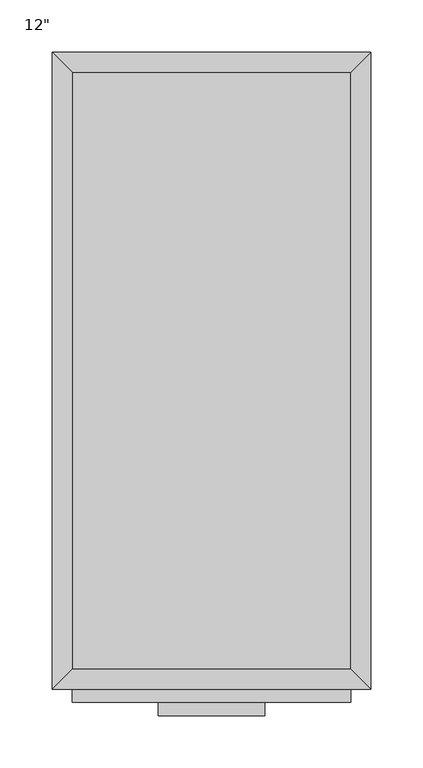
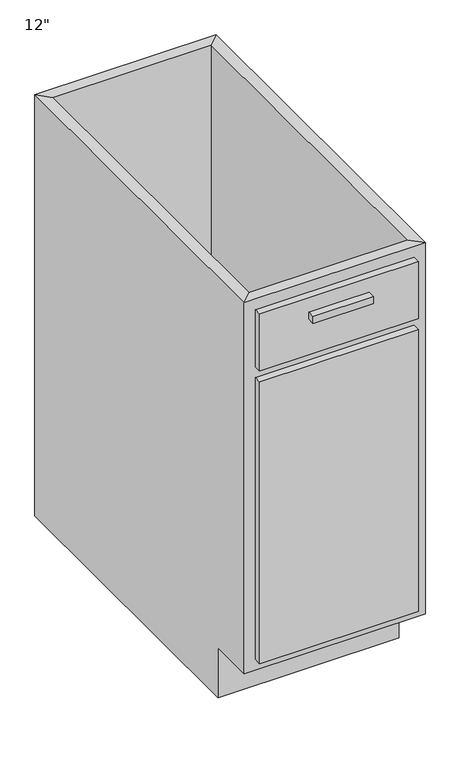
"""IFC4 building model written with IfcOpenShell, lengths in millimetres: furniture geometry."""

import ifcopenshell
import ifcopenshell.guid

model = None  # the IFC model being written
_history = None  # IfcOwnerHistory: only IFC2X3 demands one
_inside = {}  # id of a spatial element -> (the spatial element, [elements in it])
_under = {}  # id of a project, library or spatial element -> (it, [spatial elements below it])
_declared = {}  # id of a project -> (the project, [libraries it declares])
_typed = {}  # id of a type object -> (the type object, [elements of that type])
_made_of = {}  # id of a material, layer set ... -> (it, [elements and type objects made of it])


def new_model(schema):
    """Start an empty IFC model of exactly this schema.

    Asked for "IFC4X3", IfcOpenShell would pick the latest addendum, in which some entities
    have other attributes; the version numbers below select the first issue.
    IFC2X3 requires an IfcOwnerHistory on every rooted entity: one is made here for all.
    """
    global model, _history
    if schema == "IFC4X3":
        model = ifcopenshell.file(schema_version=(4, 3, 0, 0))
    else:
        model = ifcopenshell.file(schema=schema)
    _inside.clear()
    _under.clear()
    _declared.clear()
    _typed.clear()
    _made_of.clear()
    _history = None
    if model.schema == "IFC2X3":
        org = make("IfcOrganization", Name="unknown")
        user = make(
            "IfcPersonAndOrganization",
            ThePerson=make("IfcPerson", FamilyName="unknown"),
            TheOrganization=org,
        )
        app = make(
            "IfcApplication",
            ApplicationDeveloper=org,
            Version="unknown",
            ApplicationFullName="unknown",
            ApplicationIdentifier="unknown",
        )
        _history = make(
            "IfcOwnerHistory",
            OwningUser=user,
            OwningApplication=app,
            ChangeAction="ADDED",
            CreationDate=0,
        )
    return model


def make(cls, **values):
    """One entity of the class cls with the attributes given. An attribute that is None is left unset."""
    return model.create_entity(
        cls, **{name: value for name, value in values.items() if value is not None}
    )


def rooted(cls, **values):
    """An entity with a GlobalId (a new one), such as an element, a storey or a relation."""
    return make(cls, GlobalId=ifcopenshell.guid.new(), OwnerHistory=_history, **values)


def si_unit(unit_type, name, prefix=None):
    """IfcSIUnit, for example si_unit("LENGTHUNIT", "METRE", prefix="MILLI")."""
    return make("IfcSIUnit", UnitType=unit_type, Prefix=prefix, Name=name)


def assignment(units):
    """IfcUnitAssignment: the units of a project."""
    return None if units is None else make("IfcUnitAssignment", Units=units)


def point(xyz):
    """IfcCartesianPoint."""
    return None if xyz is None else make("IfcCartesianPoint", Coordinates=xyz)


def direction(xyz):
    """IfcDirection."""
    return None if xyz is None else make("IfcDirection", DirectionRatios=xyz)


def frame(location, z_axis=None, x_axis=None):
    """IfcAxis2Placement3D, a coordinate frame: its origin and axes. An axis left out is left unset."""
    return make(
        "IfcAxis2Placement3D",
        Location=point(location),
        Axis=direction(z_axis),
        RefDirection=direction(x_axis),
    )


def origin():
    """The frame at (0, 0, 0) with its axes left unset."""
    return frame((0.0, 0.0, 0.0))


def place(relative_to, where):
    """IfcLocalPlacement: puts the frame where relative to a parent placement (None: the world)."""
    return make(
        "IfcLocalPlacement", PlacementRelTo=relative_to, RelativePlacement=where
    )


def context(
    kind, dimensions, precision=None, world=None, true_north=None, identifier=None
):
    """IfcGeometricRepresentationContext, for example the 3D "Model" context."""
    return make(
        "IfcGeometricRepresentationContext",
        ContextIdentifier=identifier,
        ContextType=kind,
        CoordinateSpaceDimension=dimensions,
        Precision=precision,
        WorldCoordinateSystem=world,
        TrueNorth=true_north,
    )


def project(units=None, contexts=None):
    """IfcProject with its units and contexts."""
    return rooted(
        "IfcProject",
        Name="project",
        RepresentationContexts=contexts,
        UnitsInContext=assignment(units),
    )


def spatial(cls, under=None, at=None, **own):
    """A site, building, storey or space (cls), placed at a placement, below another one or the project."""
    s = rooted(cls, ObjectPlacement=at, **own)
    if under is not None:
        _under.setdefault(under.id(), (under, []))[1].append(s)
    return s


def polyline(points):
    """IfcPolyline through the points."""
    return make("IfcPolyline", Points=[point(p) for p in points])


def outline(outer, holes=None, kind="AREA"):
    """IfcArbitraryClosedProfileDef: a profile drawn as a closed curve; with holes, ...WithVoids."""
    if holes is None:
        return make("IfcArbitraryClosedProfileDef", ProfileType=kind, OuterCurve=outer)
    return make(
        "IfcArbitraryProfileDefWithVoids",
        ProfileType=kind,
        OuterCurve=outer,
        InnerCurves=holes,
    )


def extrude(swept, where, along, depth):
    """IfcExtrudedAreaSolid: the profile swept, set in the frame where, extruded along a direction by depth."""
    return make(
        "IfcExtrudedAreaSolid",
        SweptArea=swept,
        Position=where,
        ExtrudedDirection=direction(along),
        Depth=depth,
    )


def faces_of(points, faces, orient=None, outer=None):
    """IfcFace entities. A face is a list of loops; a loop is a list of indices into points, from 0.

    orient and outer hold one flag for each loop. By default every Orientation is true, the
    first loop of a face is its IfcFaceOuterBound and the others are IfcFaceBound.
    """
    made = []
    for i, loops in enumerate(faces):
        bounds = []
        for j, loop in enumerate(loops):
            is_outer = j == 0 if outer is None else outer[i][j]
            bounds.append(
                make(
                    "IfcFaceOuterBound" if is_outer else "IfcFaceBound",
                    Bound=make("IfcPolyLoop", Polygon=[points[k] for k in loop]),
                    Orientation=True if orient is None else orient[i][j],
                )
            )
        made.append(make("IfcFace", Bounds=bounds))
    return made


def faceted_brep(points, faces, orient=None, outer=None, voids=None):
    """IfcFacetedBrep: a solid bounded by flat faces; with voids (closed shells), ...WithVoids."""
    shared = [point(p) for p in points]
    hull = make("IfcClosedShell", CfsFaces=faces_of(shared, faces, orient, outer))
    if voids is None:
        return make("IfcFacetedBrep", Outer=hull)
    return make(
        "IfcFacetedBrepWithVoids",
        Outer=hull,
        Voids=[
            make(cls, CfsFaces=faces_of(shared, fs, o, b)) for cls, fs, o, b in voids
        ],
    )


def shape(context_of_items, identifier, shape_type, items):
    """IfcShapeRepresentation: the items that make up one representation, for example the "Body"."""
    return make(
        "IfcShapeRepresentation",
        ContextOfItems=context_of_items,
        RepresentationIdentifier=identifier,
        RepresentationType=shape_type,
        Items=items,
    )


def source(mapping_origin, context_of_items, identifier, shape_type, items):
    """IfcRepresentationMap: a shape defined once, which mapped items show again and again."""
    return make(
        "IfcRepresentationMap",
        MappingOrigin=mapping_origin,
        MappedRepresentation=shape(context_of_items, identifier, shape_type, items),
    )


def transform(
    local_origin,
    x_axis=None,
    y_axis=None,
    z_axis=None,
    scale=None,
    scale2=None,
    scale3=None,
    uniform=True,
):
    """IfcCartesianTransformationOperator3D, or its non-uniform kind. x_axis, y_axis, z_axis: its Axis1, 2, 3."""
    if uniform:
        return make(
            "IfcCartesianTransformationOperator3D",
            Axis1=direction(x_axis),
            Axis2=direction(y_axis),
            LocalOrigin=point(local_origin),
            Scale=scale,
            Axis3=direction(z_axis),
        )
    return make(
        "IfcCartesianTransformationOperator3DnonUniform",
        Axis1=direction(x_axis),
        Axis2=direction(y_axis),
        LocalOrigin=point(local_origin),
        Scale=scale,
        Axis3=direction(z_axis),
        Scale2=scale2,
        Scale3=scale3,
    )


def mapped(mapping_source, mapping_target):
    """IfcMappedItem: shows the shape of a source again, moved by a transform."""
    return make(
        "IfcMappedItem", MappingSource=mapping_source, MappingTarget=mapping_target
    )


def made_of(thing, what):
    """Note that an element or type object is made of a material, layer set ...; save() writes the relation."""
    if what is not None:
        _made_of.setdefault(what.id(), (what, []))[1].append(thing)
    return thing


def element(
    cls,
    number,
    at=None,
    inside=None,
    cuts=None,
    type_object=None,
    material=None,
    context=None,
    identifier="Body",
    shape_type=None,
    held_by="IfcProductDefinitionShape",
    body=None,
    shapes=None,
    **own,
):
    """One element of the class cls, such as IfcWall. Its Tag is "e" and its number.

    at: its placement. inside: the storey or other place that contains it. cuts: it is an
    opening in that element (IfcRelVoidsElement). A single representation is given by context,
    identifier, shape_type and body (its items); several are given by shapes. held_by: the class
    of the entity that holds the representations. save() writes the other relations.
    """
    e = rooted(cls, Tag="e%d" % number, ObjectPlacement=at, **own)
    if body is not None:
        shapes = [shape(context, identifier, shape_type, body)]
    if shapes is not None:
        e.Representation = make(held_by, Representations=shapes)
    if inside is not None:
        _inside.setdefault(inside.id(), (inside, []))[1].append(e)
    if cuts is not None:
        rooted(
            "IfcRelVoidsElement", RelatingBuildingElement=cuts, RelatedOpeningElement=e
        )
    if type_object is not None:
        _typed.setdefault(type_object.id(), (type_object, []))[1].append(e)
    return made_of(e, material)


def aggregate(whole, parts):
    """IfcRelAggregates: a whole, such as a stair, and the parts it consists of."""
    return rooted("IfcRelAggregates", RelatingObject=whole, RelatedObjects=parts)


def save(model, path):
    """Write the relations noted so far, then the file.

    IfcRelAggregates (storeys below a building ...), IfcRelContainedInSpatialStructure (elements
    in a storey), IfcRelDefinesByType, IfcRelAssociatesMaterial and IfcRelDeclares: one each for
    every whole, place, type object, material and project.
    """
    for whole, parts in _under.values():
        aggregate(whole, parts)
    for where, things in _inside.values():
        rooted(
            "IfcRelContainedInSpatialStructure",
            RelatedElements=things,
            RelatingStructure=where,
        )
    for kind, things in _typed.values():
        rooted("IfcRelDefinesByType", RelatedObjects=things, RelatingType=kind)
    for what, things in _made_of.values():
        rooted("IfcRelAssociatesMaterial", RelatedObjects=things, RelatingMaterial=what)
    for by, libraries in _declared.values():
        rooted("IfcRelDeclares", RelatingContext=by, RelatedDefinitions=libraries)
    model.write(path)


def furniture_d3494f9b(model_context):
    return source(origin(), model_context, "Body", "SolidModel", [
        faceted_brep([(152.0877049, -590.55, 749.3), (152.0877049, -590.55, 88.9), (-114.6122951, -590.55, 88.9), (-114.6122951, -590.55, 749.3), (-133.6622951, -609.6, 749.3), (171.1377049, -609.6, 749.3), (-133.6622951, -609.6, 88.9), (171.1377049, -609.6, 88.9), (-114.6122951, -533.4, 88.9), (-114.6122951, -19.05, 88.9), (-114.6122951, -19.05, 749.3), (-133.6622951, 0.0, 749.3), (-133.6622951, 0.0, 0.0), (-133.6622951, -533.4, 0.0), (-133.6622951, -533.4, 88.9), (152.0877049, -19.05, 88.9), (152.0877049, -19.05, 749.3), (171.1377049, 0.0, 749.3), (171.1377049, 0.0, 0.0), (152.0877049, -533.4, 88.9), (171.1377049, -533.4, 88.9), (171.1377049, -533.4, 0.0)], [[[0, 1, 2, 3]], [[0, 3, 4, 5]], [[5, 4, 6, 7]], [[2, 1, 7, 6]], [[3, 2, 8, 9, 10]], [[4, 3, 10, 11]], [[6, 4, 11, 12, 13, 14]], [[2, 6, 14, 8]], [[10, 9, 15, 16]], [[11, 10, 16, 17]], [[12, 11, 17, 18]], [[1, 0, 16, 15, 19]], [[0, 5, 17, 16]], [[5, 7, 20, 21, 18, 17]], [[7, 1, 19, 20]], [[8, 19, 15, 9]], [[18, 21, 13, 12]], [[13, 21, 20, 19, 8, 14]]]),
        extrude(outline(polyline([(152.0877049, -19.05), (152.0877049, -590.55), (-114.6122951, -590.55), (-114.6122951, -19.05), (152.0877049, -19.05)])), frame((0.0, 0.0, 88.9), z_axis=(0.0, 0.0, 1.0), x_axis=(1.0, 0.0, 0.0)), (0.0, 0.0, 1.0), 19.05),
        extrude(outline(polyline([(152.0877049, -622.3), (-114.6122951, -622.3), (-114.6122951, -609.6), (152.0877049, -609.6), (152.0877049, -622.3)])), frame((0.0, 0.0, 628.65), z_axis=(0.0, 0.0, 1.0), x_axis=(1.0, 0.0, 0.0)), (0.0, 0.0, 1.0), 101.6),
        extrude(outline(polyline([(152.0877049, -622.3), (-114.6122951, -622.3), (-114.6122951, -609.6), (152.0877049, -609.6), (152.0877049, -622.3)])), frame((0.0, 0.0, 107.95), z_axis=(0.0, 0.0, 1.0), x_axis=(1.0, 0.0, 0.0)), (0.0, 0.0, 1.0), 501.65),
        extrude(outline(polyline([(69.5377049, -635.0), (-32.0622951, -635.0), (-32.0622951, -622.3), (69.5377049, -622.3), (69.5377049, -635.0)])), frame((0.0, 0.0, 692.15), z_axis=(0.0, 0.0, 1.0), x_axis=(1.0, 0.0, 0.0)), (0.0, 0.0, 1.0), 12.7),
    ])


if __name__ == "__main__":
    model = new_model("IFC4")
    model_context = context("Model", 3, world=origin())
    ifc_project = project(units=[si_unit("LENGTHUNIT", "METRE", prefix="MILLI")], contexts=[model_context])
    site = spatial("IfcSite", under=ifc_project)
    building = spatial("IfcBuilding", under=site)
    placement = place(None, origin())
    furniture_shape = furniture_d3494f9b(model_context)
    element("IfcFurniture", 1, ObjectType="Vanity Cabinet-Single Door & Drawer : 12\"", at=placement, inside=building, context=model_context, shape_type="MappedRepresentation", body=[
        mapped(furniture_shape, transform((0.0, 0.0, 0.0), x_axis=(1.0, 0.0, 0.0), y_axis=(0.0, 1.0, 0.0), z_axis=(0.0, 0.0, 1.0))),
    ])
    save(model, "model.ifc")

# Revit data of these elements
# Type "Vanity Cabinet-Single Door & Drawer : 12\""
#   Assembly Code = "C1030410"
#   Depth = 2' - 0"
#   Height = 2' - 5 1/2"
#   Toe Depth = 0' - 3"
#   Toe Height = 0' - 3 1/2"
#   Width = 1' - 0"
#   Cabinet Material = none
#   Door/Drawer Material = none
#   Handle Material = Cabinets - Handles
# Element 1 (IfcFurniture, "Vanity Cabinet-Single Door & Drawer : 12\"")
#   Materials on its faces: "Cabinets", "Cabinets - Handles"
# Materials
#   "Cabinets - Handles": class "Metal", colour RGB 57 57 57, transparency 0
#   "Cabinets": class "Miscellaneous", colour RGB 249 249 249, transparency 0
